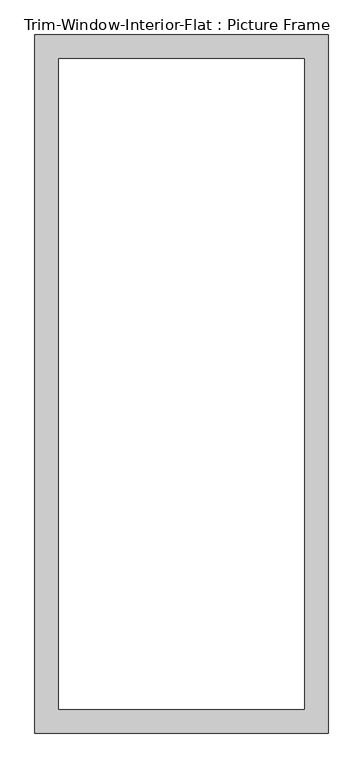
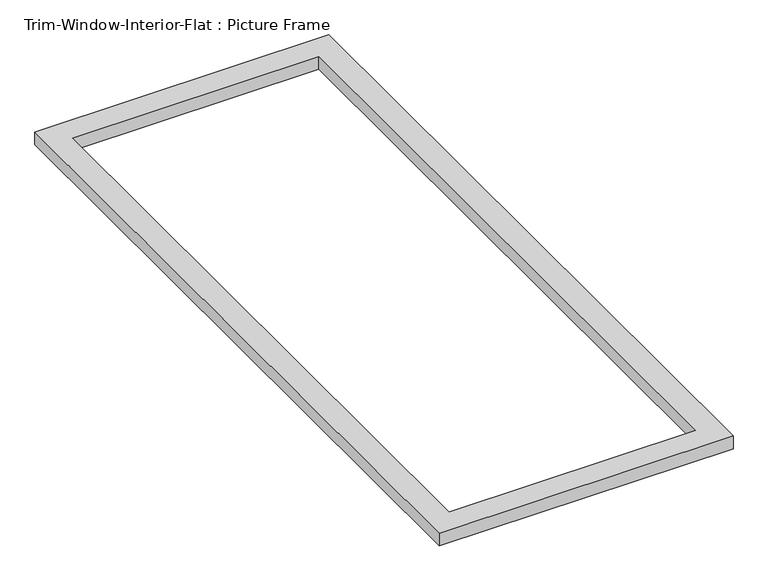
"""IFC4 building model written with IfcOpenShell, lengths in millimetres: proxy geometry, Trim-Window-Interior-Flat : Picture Frame."""

from ifc_helpers import new_model, si_unit, origin, origin_with_axes, place, context, project, spatial, polyline, outline, extrude, source, transform, mapped, element, save


def trim_window_interior_flat_picture_frame_35192fdd(model_context):
    return source(origin(), model_context, "Body", "SweptSolid", [
        extrude(outline(polyline([(349.25, 44.45), (349.25, -1619.25), (-349.25, -1619.25), (-349.25, 44.45), (349.25, 44.45)]), holes=[polyline([(292.1, -12.7), (-292.1, -12.7), (-292.1, -1562.1), (292.1, -1562.1), (292.1, -12.7)])]), origin_with_axes(), (0.0, 0.0, 1.0), 31.75),
    ])


if __name__ == "__main__":
    model = new_model("IFC4")
    model_context = context("Model", 3, world=origin())
    ifc_project = project(units=[si_unit("LENGTHUNIT", "METRE", prefix="MILLI")], contexts=[model_context])
    site = spatial("IfcSite", under=ifc_project)
    building = spatial("IfcBuilding", under=site)
    placement = place(None, origin())
    trim_window_interior_flat_picture_frame_shape = trim_window_interior_flat_picture_frame_35192fdd(model_context)
    element("IfcBuildingElementProxy", 1, Name="Trim-Window-Interior-Flat : Picture Frame", ObjectType="Trim-Window-Interior-Flat : Picture Frame", at=placement, inside=building, context=model_context, shape_type="MappedRepresentation", body=[
        mapped(trim_window_interior_flat_picture_frame_shape, transform((0.0, 0.0, 0.0), x_axis=(1.0, 0.0, 0.0), y_axis=(0.0, 1.0, 0.0), z_axis=(0.0, 0.0, 1.0))),
    ])
    save(model, "model.ifc")

# Revit data of these elements
# Type "Trim-Window-Interior-Flat : Picture Frame"
#   Trim Thickness_Picture Frame = 0' - 1 1/4"
#   Trim Width = 0' - 2 1/4"
#   Trim Thickness_with Sill = 0' - 0 3/4"
#   Sill Thickness = 0' - 1 1/4"
#   Opening Width [instance default] = 2' - 0"
#   Opening Height [instance default] = 3' - 0"
#   Default Elevation = 4' - 0"
#   Sill = no
#   Picture Frame = yes
#   Trim Material [instance default] = none
# Element 1 (IfcBuildingElementProxy, "Trim-Window-Interior-Flat : Picture Frame")
#   Opening Height = 5' - 2"
#   Trim Material = Wood - Stained
#   Materials on its faces: "Wood - Stained"
# Materials
#   "Wood - Stained": class "Wood", colour RGB 224 178 126, transparency 0, Cost = 0
